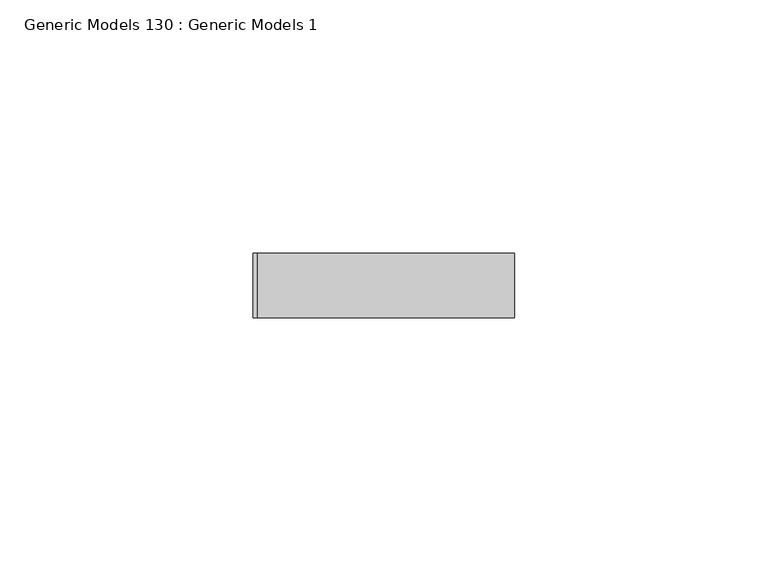
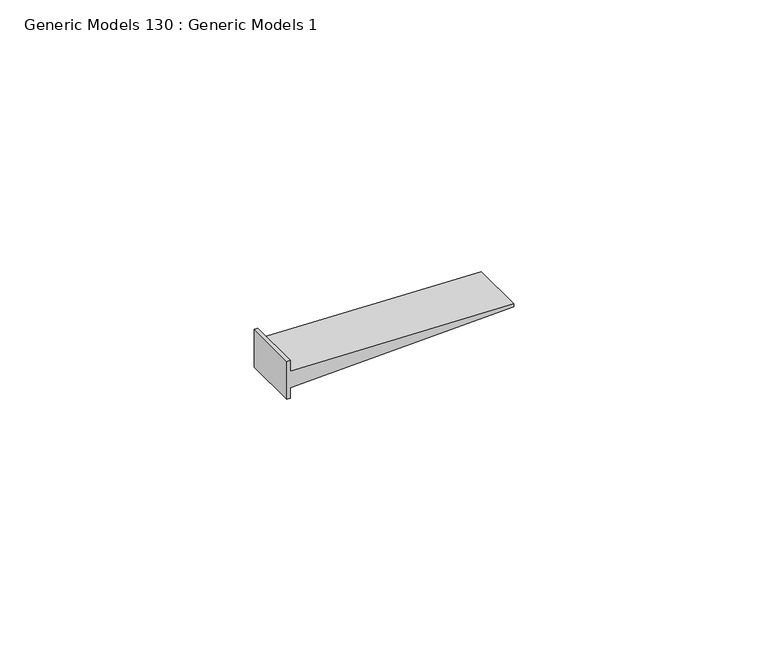
"""IFC4 building model written with IfcOpenShell, lengths in millimetres: proxy geometry, Generic Models 130 : Generic Models 1."""

from ifc_helpers import new_model, si_unit, frame, origin, place, context, project, spatial, polyline, outline, extrude, source, transform, mapped, element, save


def generic_models_130_generic_models_1_e19555d7(model_context):
    return source(origin(), model_context, "Body", "SweptSolid", [
        extrude(outline(polyline([(2183.633033, 46827.1298031), (2174.539833, 46827.1298031), (2174.539833, 46827.9235531), (2177.0896966, 46827.9235531), (2178.6870857, 46878.7235531), (2179.4857803, 46878.7235531), (2181.0831694, 46827.9235531), (2183.633033, 46827.9235531), (2183.633033, 46827.1298031)])), frame((0.0, 565.15, 0.0), z_axis=(0.0, 1.0, 0.0), x_axis=(0.0, 0.0, 1.0)), (0.0, 0.0, 1.0), 12.7),
    ])


if __name__ == "__main__":
    model = new_model("IFC4")
    model_context = context("Model", 3, world=origin())
    ifc_project = project(units=[si_unit("LENGTHUNIT", "METRE", prefix="MILLI")], contexts=[model_context])
    site = spatial("IfcSite", under=ifc_project)
    building = spatial("IfcBuilding", under=site)
    placement = place(None, origin())
    generic_models_130_generic_models_1_shape = generic_models_130_generic_models_1_e19555d7(model_context)
    element("IfcBuildingElementProxy", 1, Name="Generic Models 130 : Generic Models 1", ObjectType="Generic Models 130 : Generic Models 1", at=placement, inside=building, context=model_context, shape_type="MappedRepresentation", body=[
        mapped(generic_models_130_generic_models_1_shape, transform((0.0, 0.0, 0.0), x_axis=(1.0, 0.0, 0.0), y_axis=(0.0, 1.0, 0.0), z_axis=(0.0, 0.0, 1.0))),
    ])
    save(model, "model.ifc")

# Revit data of these elements
# Element 1 (IfcBuildingElementProxy, "Generic Models 130 : Generic Models 1")
#   Materials on its faces: "ATTACH GYPSUM BOARD TO STUDS AND NOT TO TOP TRACK"
# Materials
#   "ATTACH GYPSUM BOARD TO STUDS AND NOT TO TOP TRACK": class "Generic", colour RGB 48 48 48, transparency 0, Cost = 0
